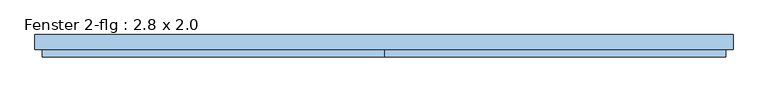
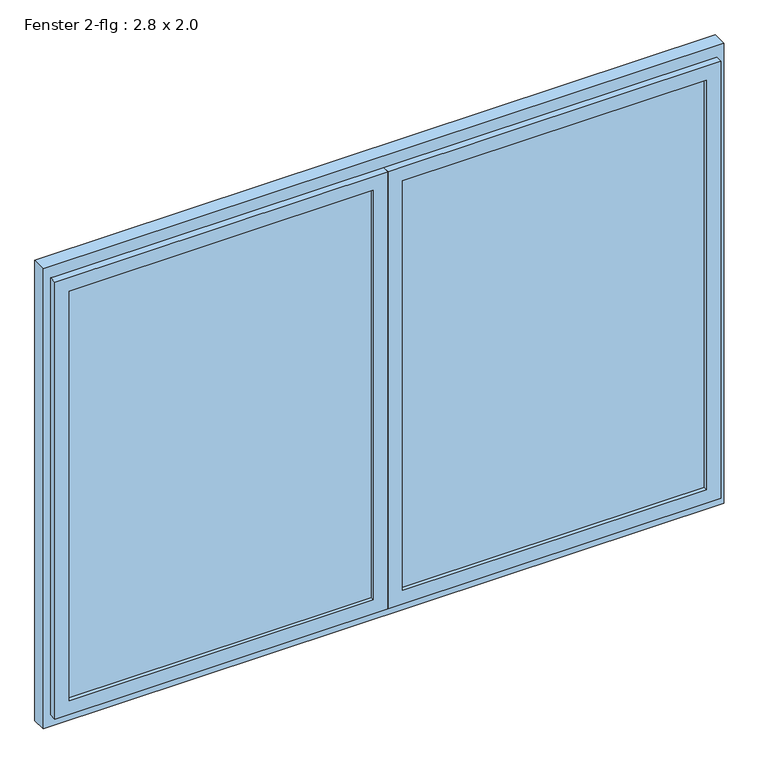
"""IFC4 building model written with IfcOpenShell, lengths in millimetres: window geometry, Fenster 2-flg : 2.8 x 2.0."""

import ifcopenshell
import ifcopenshell.guid

model = None  # the IFC model being written
_history = None  # IfcOwnerHistory: only IFC2X3 demands one
_inside = {}  # id of a spatial element -> (the spatial element, [elements in it])
_under = {}  # id of a project, library or spatial element -> (it, [spatial elements below it])
_declared = {}  # id of a project -> (the project, [libraries it declares])
_typed = {}  # id of a type object -> (the type object, [elements of that type])
_made_of = {}  # id of a material, layer set ... -> (it, [elements and type objects made of it])


def new_model(schema):
    """Start an empty IFC model of exactly this schema.

    Asked for "IFC4X3", IfcOpenShell would pick the latest addendum, in which some entities
    have other attributes; the version numbers below select the first issue.
    IFC2X3 requires an IfcOwnerHistory on every rooted entity: one is made here for all.
    """
    global model, _history
    if schema == "IFC4X3":
        model = ifcopenshell.file(schema_version=(4, 3, 0, 0))
    else:
        model = ifcopenshell.file(schema=schema)
    _inside.clear()
    _under.clear()
    _declared.clear()
    _typed.clear()
    _made_of.clear()
    _history = None
    if model.schema == "IFC2X3":
        org = make("IfcOrganization", Name="unknown")
        user = make(
            "IfcPersonAndOrganization",
            ThePerson=make("IfcPerson", FamilyName="unknown"),
            TheOrganization=org,
        )
        app = make(
            "IfcApplication",
            ApplicationDeveloper=org,
            Version="unknown",
            ApplicationFullName="unknown",
            ApplicationIdentifier="unknown",
        )
        _history = make(
            "IfcOwnerHistory",
            OwningUser=user,
            OwningApplication=app,
            ChangeAction="ADDED",
            CreationDate=0,
        )
    return model


def make(cls, **values):
    """One entity of the class cls with the attributes given. An attribute that is None is left unset."""
    return model.create_entity(
        cls, **{name: value for name, value in values.items() if value is not None}
    )


def rooted(cls, **values):
    """An entity with a GlobalId (a new one), such as an element, a storey or a relation."""
    return make(cls, GlobalId=ifcopenshell.guid.new(), OwnerHistory=_history, **values)


def si_unit(unit_type, name, prefix=None):
    """IfcSIUnit, for example si_unit("LENGTHUNIT", "METRE", prefix="MILLI")."""
    return make("IfcSIUnit", UnitType=unit_type, Prefix=prefix, Name=name)


def assignment(units):
    """IfcUnitAssignment: the units of a project."""
    return None if units is None else make("IfcUnitAssignment", Units=units)


def point(xyz):
    """IfcCartesianPoint."""
    return None if xyz is None else make("IfcCartesianPoint", Coordinates=xyz)


def direction(xyz):
    """IfcDirection."""
    return None if xyz is None else make("IfcDirection", DirectionRatios=xyz)


def frame(location, z_axis=None, x_axis=None):
    """IfcAxis2Placement3D, a coordinate frame: its origin and axes. An axis left out is left unset."""
    return make(
        "IfcAxis2Placement3D",
        Location=point(location),
        Axis=direction(z_axis),
        RefDirection=direction(x_axis),
    )


def origin():
    """The frame at (0, 0, 0) with its axes left unset."""
    return frame((0.0, 0.0, 0.0))


def place(relative_to, where):
    """IfcLocalPlacement: puts the frame where relative to a parent placement (None: the world)."""
    return make(
        "IfcLocalPlacement", PlacementRelTo=relative_to, RelativePlacement=where
    )


def context(
    kind, dimensions, precision=None, world=None, true_north=None, identifier=None
):
    """IfcGeometricRepresentationContext, for example the 3D "Model" context."""
    return make(
        "IfcGeometricRepresentationContext",
        ContextIdentifier=identifier,
        ContextType=kind,
        CoordinateSpaceDimension=dimensions,
        Precision=precision,
        WorldCoordinateSystem=world,
        TrueNorth=true_north,
    )


def project(units=None, contexts=None):
    """IfcProject with its units and contexts."""
    return rooted(
        "IfcProject",
        Name="project",
        RepresentationContexts=contexts,
        UnitsInContext=assignment(units),
    )


def spatial(cls, under=None, at=None, **own):
    """A site, building, storey or space (cls), placed at a placement, below another one or the project."""
    s = rooted(cls, ObjectPlacement=at, **own)
    if under is not None:
        _under.setdefault(under.id(), (under, []))[1].append(s)
    return s


def polyline(points):
    """IfcPolyline through the points."""
    return make("IfcPolyline", Points=[point(p) for p in points])


def outline(outer, holes=None, kind="AREA"):
    """IfcArbitraryClosedProfileDef: a profile drawn as a closed curve; with holes, ...WithVoids."""
    if holes is None:
        return make("IfcArbitraryClosedProfileDef", ProfileType=kind, OuterCurve=outer)
    return make(
        "IfcArbitraryProfileDefWithVoids",
        ProfileType=kind,
        OuterCurve=outer,
        InnerCurves=holes,
    )


def extrude(swept, where, along, depth):
    """IfcExtrudedAreaSolid: the profile swept, set in the frame where, extruded along a direction by depth."""
    return make(
        "IfcExtrudedAreaSolid",
        SweptArea=swept,
        Position=where,
        ExtrudedDirection=direction(along),
        Depth=depth,
    )


def faces_of(points, faces, orient=None, outer=None):
    """IfcFace entities. A face is a list of loops; a loop is a list of indices into points, from 0.

    orient and outer hold one flag for each loop. By default every Orientation is true, the
    first loop of a face is its IfcFaceOuterBound and the others are IfcFaceBound.
    """
    made = []
    for i, loops in enumerate(faces):
        bounds = []
        for j, loop in enumerate(loops):
            is_outer = j == 0 if outer is None else outer[i][j]
            bounds.append(
                make(
                    "IfcFaceOuterBound" if is_outer else "IfcFaceBound",
                    Bound=make("IfcPolyLoop", Polygon=[points[k] for k in loop]),
                    Orientation=True if orient is None else orient[i][j],
                )
            )
        made.append(make("IfcFace", Bounds=bounds))
    return made


def faceted_brep(points, faces, orient=None, outer=None, voids=None):
    """IfcFacetedBrep: a solid bounded by flat faces; with voids (closed shells), ...WithVoids."""
    shared = [point(p) for p in points]
    hull = make("IfcClosedShell", CfsFaces=faces_of(shared, faces, orient, outer))
    if voids is None:
        return make("IfcFacetedBrep", Outer=hull)
    return make(
        "IfcFacetedBrepWithVoids",
        Outer=hull,
        Voids=[
            make(cls, CfsFaces=faces_of(shared, fs, o, b)) for cls, fs, o, b in voids
        ],
    )


def shape(context_of_items, identifier, shape_type, items):
    """IfcShapeRepresentation: the items that make up one representation, for example the "Body"."""
    return make(
        "IfcShapeRepresentation",
        ContextOfItems=context_of_items,
        RepresentationIdentifier=identifier,
        RepresentationType=shape_type,
        Items=items,
    )


def source(mapping_origin, context_of_items, identifier, shape_type, items):
    """IfcRepresentationMap: a shape defined once, which mapped items show again and again."""
    return make(
        "IfcRepresentationMap",
        MappingOrigin=mapping_origin,
        MappedRepresentation=shape(context_of_items, identifier, shape_type, items),
    )


def transform(
    local_origin,
    x_axis=None,
    y_axis=None,
    z_axis=None,
    scale=None,
    scale2=None,
    scale3=None,
    uniform=True,
):
    """IfcCartesianTransformationOperator3D, or its non-uniform kind. x_axis, y_axis, z_axis: its Axis1, 2, 3."""
    if uniform:
        return make(
            "IfcCartesianTransformationOperator3D",
            Axis1=direction(x_axis),
            Axis2=direction(y_axis),
            LocalOrigin=point(local_origin),
            Scale=scale,
            Axis3=direction(z_axis),
        )
    return make(
        "IfcCartesianTransformationOperator3DnonUniform",
        Axis1=direction(x_axis),
        Axis2=direction(y_axis),
        LocalOrigin=point(local_origin),
        Scale=scale,
        Axis3=direction(z_axis),
        Scale2=scale2,
        Scale3=scale3,
    )


def mapped(mapping_source, mapping_target):
    """IfcMappedItem: shows the shape of a source again, moved by a transform."""
    return make(
        "IfcMappedItem", MappingSource=mapping_source, MappingTarget=mapping_target
    )


def made_of(thing, what):
    """Note that an element or type object is made of a material, layer set ...; save() writes the relation."""
    if what is not None:
        _made_of.setdefault(what.id(), (what, []))[1].append(thing)
    return thing


def element(
    cls,
    number,
    at=None,
    inside=None,
    cuts=None,
    type_object=None,
    material=None,
    context=None,
    identifier="Body",
    shape_type=None,
    held_by="IfcProductDefinitionShape",
    body=None,
    shapes=None,
    **own,
):
    """One element of the class cls, such as IfcWall. Its Tag is "e" and its number.

    at: its placement. inside: the storey or other place that contains it. cuts: it is an
    opening in that element (IfcRelVoidsElement). A single representation is given by context,
    identifier, shape_type and body (its items); several are given by shapes. held_by: the class
    of the entity that holds the representations. save() writes the other relations.
    """
    e = rooted(cls, Tag="e%d" % number, ObjectPlacement=at, **own)
    if body is not None:
        shapes = [shape(context, identifier, shape_type, body)]
    if shapes is not None:
        e.Representation = make(held_by, Representations=shapes)
    if inside is not None:
        _inside.setdefault(inside.id(), (inside, []))[1].append(e)
    if cuts is not None:
        rooted(
            "IfcRelVoidsElement", RelatingBuildingElement=cuts, RelatedOpeningElement=e
        )
    if type_object is not None:
        _typed.setdefault(type_object.id(), (type_object, []))[1].append(e)
    return made_of(e, material)


def aggregate(whole, parts):
    """IfcRelAggregates: a whole, such as a stair, and the parts it consists of."""
    return rooted("IfcRelAggregates", RelatingObject=whole, RelatedObjects=parts)


def save(model, path):
    """Write the relations noted so far, then the file.

    IfcRelAggregates (storeys below a building ...), IfcRelContainedInSpatialStructure (elements
    in a storey), IfcRelDefinesByType, IfcRelAssociatesMaterial and IfcRelDeclares: one each for
    every whole, place, type object, material and project.
    """
    for whole, parts in _under.values():
        aggregate(whole, parts)
    for where, things in _inside.values():
        rooted(
            "IfcRelContainedInSpatialStructure",
            RelatedElements=things,
            RelatingStructure=where,
        )
    for kind, things in _typed.values():
        rooted("IfcRelDefinesByType", RelatedObjects=things, RelatingType=kind)
    for what, things in _made_of.values():
        rooted("IfcRelAssociatesMaterial", RelatedObjects=things, RelatingMaterial=what)
    for by, libraries in _declared.values():
        rooted("IfcRelDeclares", RelatingContext=by, RelatedDefinitions=libraries)
    model.write(path)


def fenster_2_flg_2_8_x_2_0_ff653881(model_context):
    return source(origin(), model_context, "Body", "SolidModel", [
        extrude(outline(polyline([(30.0, -15.0), (-30.0, -15.0), (-30.0, 45.0), (30.0, 45.0), (30.0, -15.0)])), frame((0.0, 0.0, 1080.0), z_axis=(0.0, 0.0, 1.0), x_axis=(1.0, 0.0, 0.0)), (0.0, 0.0, 1.0), 1840.0),
        extrude(outline(polyline([(3000.0, -1400.0), (1000.0, -1400.0), (1000.0, 1400.0), (3000.0, 1400.0), (3000.0, -1400.0)]), holes=[polyline([(2920.0, -1340.0), (2920.0, 1340.0), (1080.0, 1340.0), (1080.0, -1340.0), (2920.0, -1340.0)])]), frame((0.0, -15.0, 0.0), z_axis=(0.0, 1.0, 0.0), x_axis=(0.0, 0.0, 1.0)), (0.0, 0.0, 1.0), 60.0),
        faceted_brep([(-1340.0, -15.0, 1080.0), (-1340.0, 15.0, 1080.0), (-30.0, 15.0, 1080.0), (-30.0, -15.0, 1080.0), (-30.0, 15.0, 2920.0), (-30.0, -15.0, 2920.0), (-1340.0, 15.0, 2920.0), (-60.0, 15.0, 2890.0), (-1310.0, 15.0, 2890.0), (-1310.0, 15.0, 1110.0), (-60.0, 15.0, 1110.0), (0.0, -15.0, 1050.0), (-1370.0, -15.0, 1050.0), (-1370.0, -15.0, 2950.0), (0.0, -15.0, 2950.0), (-1340.0, -15.0, 2920.0), (-1370.0, -45.0, 1050.0), (0.0, -45.0, 1050.0), (0.0, -45.0, 2950.0), (-1370.0, -45.0, 2950.0), (-60.0, -45.0, 1110.0), (-1310.0, -45.0, 1110.0), (-1310.0, -45.0, 2890.0), (-60.0, -45.0, 2890.0)], [[[0, 1, 2, 3]], [[3, 2, 4, 5]], [[2, 1, 6, 4], [7, 8, 9, 10]], [[11, 12, 13, 14], [5, 15, 0, 3]], [[16, 12, 11, 17]], [[17, 11, 14, 18]], [[18, 19, 16, 17], [20, 21, 22, 23]], [[9, 21, 20, 10]], [[10, 20, 23, 7]], [[15, 6, 1, 0]], [[19, 13, 12, 16]], [[8, 22, 21, 9]], [[5, 4, 6, 15]], [[18, 14, 13, 19]], [[7, 23, 22, 8]]]),
        faceted_brep([(30.0, -15.0, 1080.0), (30.0, 15.0, 1080.0), (1340.0, 15.0, 1080.0), (1340.0, -15.0, 1080.0), (1340.0, 15.0, 2920.0), (1340.0, -15.0, 2920.0), (30.0, 15.0, 2920.0), (1310.0, 15.0, 2890.0), (60.0, 15.0, 2890.0), (60.0, 15.0, 1110.0), (1310.0, 15.0, 1110.0), (1370.0, -15.0, 1050.0), (0.0, -15.0, 1050.0), (0.0, -15.0, 2950.0), (1370.0, -15.0, 2950.0), (30.0, -15.0, 2920.0), (0.0, -45.0, 1050.0), (1370.0, -45.0, 1050.0), (1370.0, -45.0, 2950.0), (0.0, -45.0, 2950.0), (1310.0, -45.0, 1110.0), (60.0, -45.0, 1110.0), (60.0, -45.0, 2890.0), (1310.0, -45.0, 2890.0)], [[[0, 1, 2, 3]], [[3, 2, 4, 5]], [[2, 1, 6, 4], [7, 8, 9, 10]], [[11, 12, 13, 14], [5, 15, 0, 3]], [[16, 12, 11, 17]], [[17, 11, 14, 18]], [[18, 19, 16, 17], [20, 21, 22, 23]], [[9, 21, 20, 10]], [[10, 20, 23, 7]], [[15, 6, 1, 0]], [[19, 13, 12, 16]], [[8, 22, 21, 9]], [[5, 4, 6, 15]], [[18, 14, 13, 19]], [[7, 23, 22, 8]]]),
        extrude(outline(polyline([(60.0, 0.0), (1310.0, 0.0), (1310.0, -30.0), (60.0, -30.0), (60.0, 0.0)])), frame((0.0, 0.0, 1110.0), z_axis=(0.0, 0.0, 1.0), x_axis=(1.0, 0.0, 0.0)), (0.0, 0.0, 1.0), 1780.0),
        extrude(outline(polyline([(-1310.0, 0.0), (-60.0, 0.0), (-60.0, -30.0), (-1310.0, -30.0), (-1310.0, 0.0)])), frame((0.0, 0.0, 1110.0), z_axis=(0.0, 0.0, 1.0), x_axis=(1.0, 0.0, 0.0)), (0.0, 0.0, 1.0), 1780.0),
    ])


if __name__ == "__main__":
    model = new_model("IFC4")
    model_context = context("Model", 3, world=origin())
    ifc_project = project(units=[si_unit("LENGTHUNIT", "METRE", prefix="MILLI")], contexts=[model_context])
    site = spatial("IfcSite", under=ifc_project)
    building = spatial("IfcBuilding", under=site)
    placement = place(None, origin())
    fenster_2_flg_2_8_x_2_0_shape = fenster_2_flg_2_8_x_2_0_ff653881(model_context)
    element("IfcWindow", 1, ObjectType="Fenster 2-flg : 2.8 x 2.0", at=placement, inside=building, context=model_context, shape_type="MappedRepresentation", body=[
        mapped(fenster_2_flg_2_8_x_2_0_shape, transform((0.0, 0.0, 0.0), x_axis=(1.0, 0.0, 0.0), y_axis=(0.0, 1.0, 0.0), z_axis=(0.0, 0.0, 1.0))),
    ])
    save(model, "model.ifc")

# Revit data of these elements
# Type "Fenster 2-flg : 2.8 x 2.0"
#   Type Mark = "77"
#   Operation = "DoublePanelVertical"
#   Keynote = "16.05.01"
#   Visual Light Transmittance = 0.9
#   Solar Heat Gain Coefficient = 0.78
#   Rough Width = 2.800 m
#   Rough Height = 2.000 m
#   Heat Transfer Coefficient (U) = 3.6886 W/(m²·K)
#   Rahmentiefe = 0.060 m
#   Rahmenhöhe unten = 0.080 m
#   Höhe oberer  Rahmen = 0.080 m
#   Rahmenbreite = 0.060 m
#   Height = 2.000 m
#   Tiefe Flügel = 0.060 m
#   Flügelbreite = 0.060 m
#   Einbautiefe (von außen) [instance default] = 0.140 m
#   Width = 2.800 m
#   Öffnungsrichtung oben [instance default] = yes
#   Öffnungsrichtung in Draufsicht anzeigen [instance default] = no
#   Drehflügel 1 [instance default] = yes
#   Bild [instance default] = none
#   Glas [instance default] = none
#   Fensterflügel [instance default] = none
#   Äußere Fensterbank [instance default] = none
#   Innere Fensterbank [instance default] = none
#   Construction Type Id = ""
#   Wall Closure = (empty or 0)
#   Analytic Construction = (empty or 0)
# Element 1 (IfcWindow, "Fenster 2-flg : 2.8 x 2.0")
#   Einbautiefe (von außen) = 0.230 m
#   Materials on its faces: "Kunststoff - Weiß", "Glas"
# Materials
#   "Kunststoff - Weiß": class "Kunststoff", colour RGB 249 249 249, transparency 0, Cost = 0
#   "Glas": class "Glas", colour RGB 0 0 255, transparency 0.75, Comments = "Render-Darstellung nicht aktualisiert ", Cost = 0
